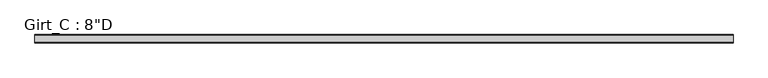
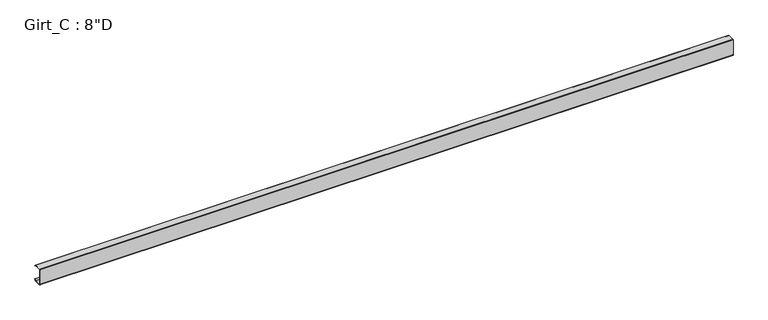
"""IFC4 building model written with IfcOpenShell, lengths in millimetres: beam geometry."""

from ifc_helpers import new_model, si_unit, point, frame, frame_2d, origin, place, context, project, spatial, polyline, circle_curve, trimmed, segment, composite_curve, outline, extrude, source, transform, mapped, element, save


def beam_a1f81ca6(model_context):
    return source(origin(), model_context, "Body", "SweptSolid", [
        extrude(outline(composite_curve([segment(polyline([(87.5109375, 101.6), (99.7560415, 87.0068534), (97.6278742, 85.221109), (86.2154765, 98.821875), (3.3005807, 98.821875)]), True, "CONTINUOUS"), segment(trimmed(circle_curve(frame_2d((3.3741066, 96.8381931)), 1.9850441), [point((3.3005807, 98.821875))], [point((1.3890625, 96.8381931))], True, "CARTESIAN"), True, "CONTINUOUS"), segment(polyline([(1.3890625, 96.8381931), (1.3890625, -96.8389339)]), True, "CONTINUOUS"), segment(trimmed(circle_curve(frame_2d((3.3748024, -96.8389339)), 1.9857399), [point((1.3890625, -96.8389339))], [point((3.2694106, -98.821875))], True, "CARTESIAN"), True, "CONTINUOUS"), segment(polyline([(3.2694106, -98.821875), (86.2154765, -98.821875), (97.6510975, -85.1934327), (99.7792647, -86.979177), (87.5109375, -101.6), (3.3734375, -101.6)]), True, "CONTINUOUS"), segment(trimmed(circle_curve(frame_2d((3.3734375, -96.8375)), 4.7625), [point((3.3734375, -101.6))], [point((-1.3890625, -96.8375))], False, "CARTESIAN"), True, "CONTINUOUS"), segment(polyline([(-1.3890625, -96.8375), (-1.3890625, 96.8375)]), True, "CONTINUOUS"), segment(trimmed(circle_curve(frame_2d((3.3734375, 96.8375)), 4.7625), [point((-1.3890625, 96.8375))], [point((3.3734375, 101.6))], False, "CARTESIAN"), True, "CONTINUOUS"), segment(polyline([(3.3734375, 101.6), (87.5109375, 101.6)]), True, "CONTINUOUS")], self_intersect=False)), frame((-4281.4875, 0.0, 0.0), z_axis=(1.0, 0.0, 0.0), x_axis=(0.0, 1.0, 0.0)), (0.0, 0.0, 1.0), 8562.975),
    ])


if __name__ == "__main__":
    model = new_model("IFC4")
    model_context = context("Model", 3, world=origin())
    ifc_project = project(units=[si_unit("LENGTHUNIT", "METRE", prefix="MILLI")], contexts=[model_context])
    site = spatial("IfcSite", under=ifc_project)
    building = spatial("IfcBuilding", under=site)
    placement = place(None, origin())
    beam_shape = beam_a1f81ca6(model_context)
    element("IfcBeam", 1, ObjectType="Girt_C : 8\"D", at=placement, inside=building, context=model_context, shape_type="MappedRepresentation", body=[
        mapped(beam_shape, transform((0.0, 0.0, 0.0), x_axis=(1.0, 0.0, 0.0), y_axis=(0.0, 1.0, 0.0), z_axis=(0.0, 0.0, 1.0))),
    ])
    save(model, "model.ifc")

# Revit data of these elements
# Type "Girt_C : 8\"D"
#   half leg = 0' - 1 3/4"
#   Web_Thickness = 0' - 0 7/64"
#   Length [instance default] = 10' - 0"
#   Leg_1 = 0' - 3 1/2"
#   Height = 0' - 8"
#   Structural Material [instance default] = none
# Element 1 (IfcBeam, "Girt_C : 8\"D")
#   Structural Material = GALVANIZED 'CEE' SECTION (8.0x3.5C - SEE STRUCT. DWGS)
#   Materials on its faces: "GALVANIZED 'CEE' SECTION (8.0x3.5C - SEE STRUCT. DWGS)"
# Materials
#   "GALVANIZED 'CEE' SECTION (8.0x3.5C - SEE STRUCT. DWGS)": class "Metal", colour RGB 137 146 153, transparency 0, Description = "Steel, mill finish", Cost = 0
